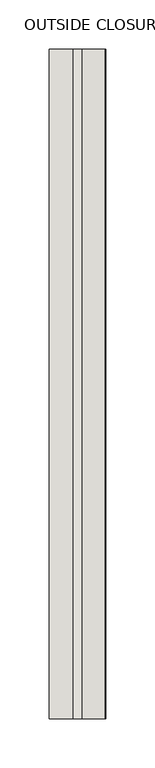
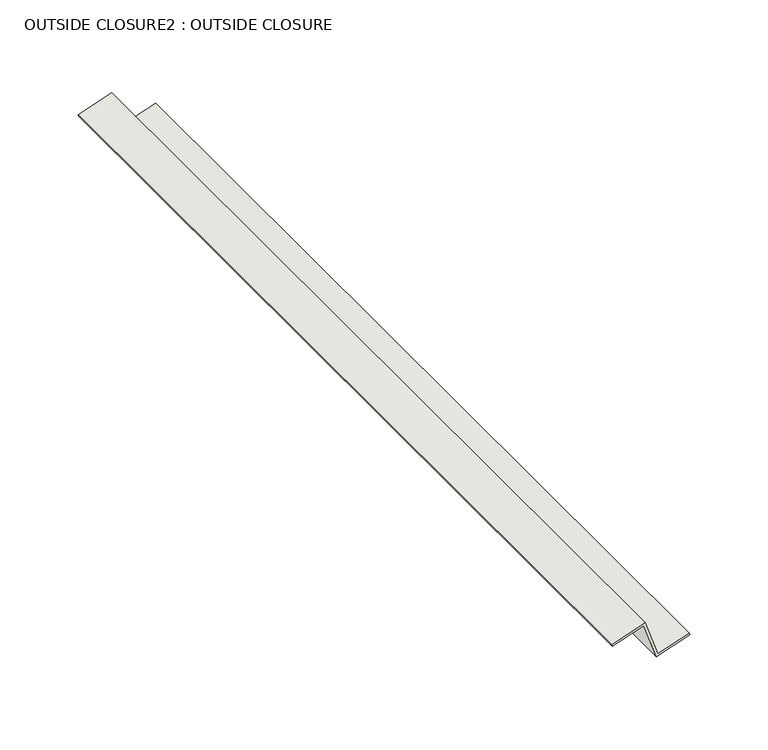
"""IFC4 building model written with IfcOpenShell, lengths in millimetres: wall geometry, OUTSIDE CLOSURE2 : OUTSIDE CLOSURE."""

from ifc_helpers import new_model, si_unit, frame, origin, place, context, project, spatial, polyline, outline, extrude, source, transform, mapped, element, save


def outside_closure2_outside_closure_554aa1ed(model_context):
    return source(origin(), model_context, "Body", "SweptSolid", [
        extrude(outline(polyline([(5859.8565193, 21321.4742997), (5858.3511446, 21321.978287), (5866.1629485, 21345.3115949), (5839.0272141, 21354.3964207), (5847.3430053, 21379.2351033), (5848.8746563, 21378.7223188), (5841.0628524, 21355.3890109), (5868.1723106, 21346.3129823), (5859.8565193, 21321.4742997)])), frame((0.0, -2319.6634634, 0.0), z_axis=(0.0, 1.0, 0.0), x_axis=(0.0, 0.0, 1.0)), (0.0, 0.0, 1.0), 682.625),
    ])


if __name__ == "__main__":
    model = new_model("IFC4")
    model_context = context("Model", 3, world=origin())
    ifc_project = project(units=[si_unit("LENGTHUNIT", "METRE", prefix="MILLI")], contexts=[model_context])
    site = spatial("IfcSite", under=ifc_project)
    building = spatial("IfcBuilding", under=site)
    placement = place(None, origin())
    outside_closure2_outside_closure_shape = outside_closure2_outside_closure_554aa1ed(model_context)
    element("IfcWall", 1, ObjectType="OUTSIDE CLOSURE2 : OUTSIDE CLOSURE", at=placement, inside=building, context=model_context, shape_type="MappedRepresentation", body=[
        mapped(outside_closure2_outside_closure_shape, transform((0.0, 0.0, 0.0), x_axis=(1.0, 0.0, 0.0), y_axis=(0.0, 1.0, 0.0), z_axis=(0.0, 0.0, 1.0))),
    ])
    save(model, "model.ifc")

# Revit data of these elements
# Element 1 (IfcWall, "OUTSIDE CLOSURE2 : OUTSIDE CLOSURE")
#   Materials on its faces: "OUTSIDE CLOSURE"
# Materials
#   "OUTSIDE CLOSURE": class "Metal", colour RGB 247 247 247, transparency 0, Cost = 0
